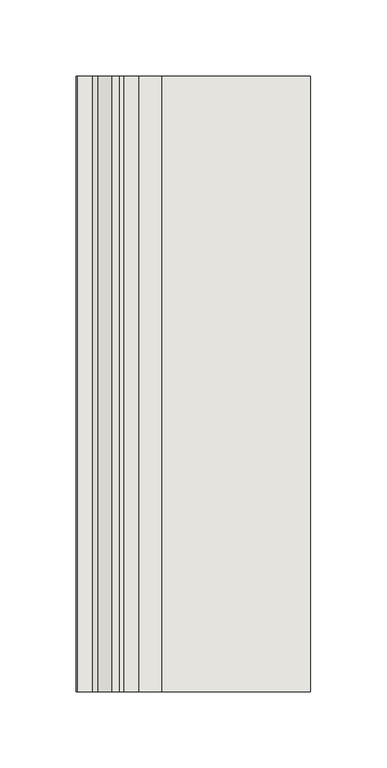
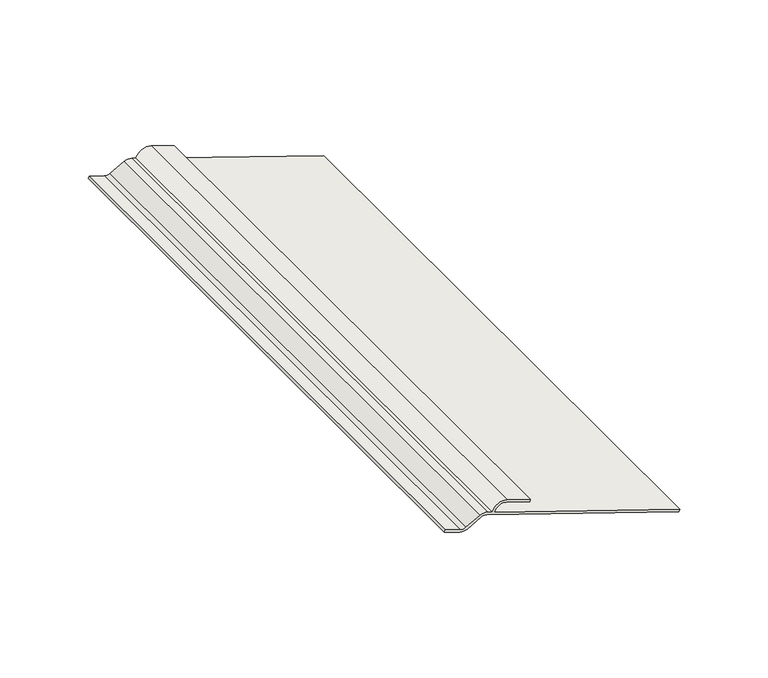
"""IFC4 building model written with IfcOpenShell, lengths in millimetres: wall geometry, BACKUP PLATE1 : BACKUP PLATE."""

from ifc_helpers import new_model, si_unit, point, frame, frame_2d, origin, place, context, project, spatial, polyline, circle_curve, trimmed, segment, composite_curve, outline, extrude, source, transform, mapped, element, save


def wall_27a8e094(model_context):
    return source(origin(), model_context, "Body", "SweptSolid", [
        extrude(outline(composite_curve([segment(polyline([(5867.3970481, 21484.547274), (5862.1682866, 21475.1350339)]), True, "CONTINUOUS"), segment(trimmed(circle_curve(frame_2d((5866.4307872, 21473.0107705)), 4.7625), [point((5862.1682866, 21475.1350339))], [point((5861.9146631, 21471.4988085))], True, "CARTESIAN"), True, "CONTINUOUS"), segment(polyline([(5861.9146631, 21471.4988085), (5865.2429702, 21461.5573895), (5863.8026277, 21461.0751744), (5860.4743205, 21471.0165934)]), True, "CONTINUOUS"), segment(trimmed(circle_curve(frame_2d((5866.4307872, 21473.0107705)), 6.28142), [point((5860.4743205, 21471.0165934))], [point((5860.8088331, 21475.8125323))], False, "CARTESIAN"), True, "CONTINUOUS"), segment(polyline([(5860.8088331, 21475.8125323), (5866.0375946, 21485.2247724)]), True, "CONTINUOUS"), segment(trimmed(circle_curve(frame_2d((5861.775094, 21487.3490358)), 4.7625), [point((5866.0375946, 21485.2247724))], [point((5866.2912181, 21488.8609978))], True, "CARTESIAN"), True, "CONTINUOUS"), segment(polyline([(5866.2912181, 21488.8609978), (5824.2479322, 21614.4413314), (5825.6882747, 21614.9235465), (5866.2781075, 21493.684575)]), True, "CONTINUOUS"), segment(trimmed(circle_curve(frame_2d((5864.3329451, 21499.7810134)), 6.3992358), [point((5866.2781075, 21493.684575))], [point((5870.4604125, 21501.6261043))], True, "CARTESIAN"), True, "CONTINUOUS"), segment(polyline([(5870.4604125, 21501.6261043), (5865.3987668, 21516.7448835), (5866.8391093, 21517.2270986), (5871.9007551, 21502.1083194)]), True, "CONTINUOUS"), segment(trimmed(circle_curve(frame_2d((5864.4121733, 21499.7610302)), 7.8478419), [point((5871.9007551, 21502.1083194))], [point((5866.7516902, 21492.2700167))], False, "CARTESIAN"), True, "CONTINUOUS"), segment(polyline([(5866.7516902, 21492.2700167), (5867.7315606, 21489.3432129)]), True, "CONTINUOUS"), segment(trimmed(circle_curve(frame_2d((5861.775094, 21487.3490358)), 6.28142), [point((5867.7315606, 21489.3432129))], [point((5867.3970481, 21484.547274))], False, "CARTESIAN"), True, "CONTINUOUS")], self_intersect=False)), frame((0.0, -1256.0384634, 0.0), z_axis=(0.0, 1.0, 0.0), x_axis=(0.0, 0.0, 1.0)), (0.0, 0.0, 1.0), 403.4547326),
    ])


if __name__ == "__main__":
    model = new_model("IFC4")
    model_context = context("Model", 3, world=origin())
    ifc_project = project(units=[si_unit("LENGTHUNIT", "METRE", prefix="MILLI")], contexts=[model_context])
    site = spatial("IfcSite", under=ifc_project)
    building = spatial("IfcBuilding", under=site)
    placement = place(None, origin())
    wall_shape = wall_27a8e094(model_context)
    element("IfcWall", 1, ObjectType="BACKUP PLATE1 : BACKUP PLATE", at=placement, inside=building, context=model_context, shape_type="MappedRepresentation", body=[
        mapped(wall_shape, transform((0.0, 0.0, 0.0), x_axis=(1.0, 0.0, 0.0), y_axis=(0.0, 1.0, 0.0), z_axis=(0.0, 0.0, 1.0))),
    ])
    save(model, "model.ifc")

# Revit data of these elements
# Element 1 (IfcWall, "BACKUP PLATE1 : BACKUP PLATE")
#   Materials on its faces: "BACKUP PLATE"
# Materials
#   "BACKUP PLATE": class "Generic", colour RGB 195 195 195, transparency 0, Cost = 0
